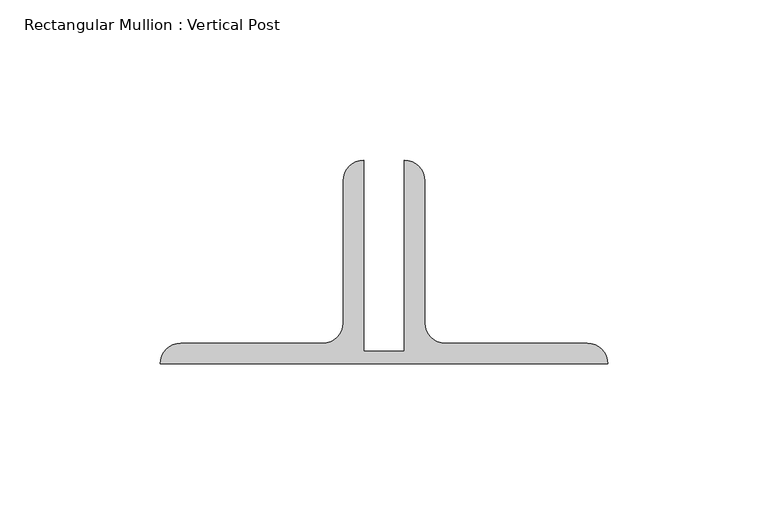
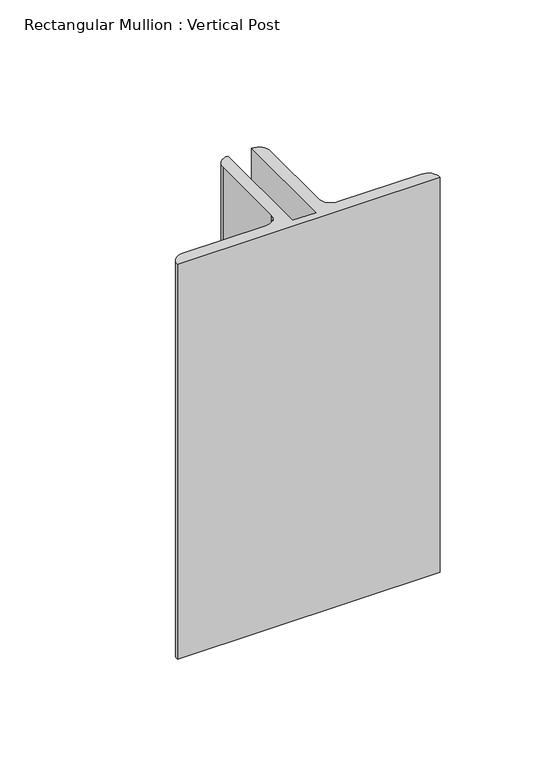
"""IFC4 building model written with IfcOpenShell, lengths in millimetres: member geometry, Rectangular Mullion : Vertical Post."""

from ifc_helpers import new_model, si_unit, point, frame, frame_2d, origin, place, context, project, spatial, polyline, circle_curve, trimmed, segment, composite_curve, outline, extrude, source, transform, mapped, element, save


def rectangular_mullion_vertical_post_d81d6a22(model_context):
    return source(origin(), model_context, "Body", "SweptSolid", [
        extrude(outline(composite_curve([segment(polyline([(-6.35, 22.9145205), (6.35, 22.9145205), (6.35, 82.55)]), True, "CONTINUOUS"), segment(trimmed(circle_curve(frame_2d((6.35, 76.2)), 6.35), [point((6.35, 82.55))], [point((12.7, 76.2))], False, "CARTESIAN"), True, "CONTINUOUS"), segment(polyline([(12.7, 76.2), (12.7, 31.75)]), True, "CONTINUOUS"), segment(trimmed(circle_curve(frame_2d((19.05, 31.75)), 6.35), [point((12.7, 31.75))], [point((19.05, 25.4))], True, "CARTESIAN"), True, "CONTINUOUS"), segment(polyline([(19.05, 25.4), (63.5, 25.4)]), True, "CONTINUOUS"), segment(trimmed(circle_curve(frame_2d((63.5, 19.05)), 6.35), [point((63.5, 25.4))], [point((69.85, 19.05))], False, "CARTESIAN"), True, "CONTINUOUS"), segment(polyline([(69.85, 19.05), (-69.85, 19.05)]), True, "CONTINUOUS"), segment(trimmed(circle_curve(frame_2d((-63.5, 19.05)), 6.35), [point((-69.85, 19.05))], [point((-63.5, 25.4))], False, "CARTESIAN"), True, "CONTINUOUS"), segment(polyline([(-63.5, 25.4), (-19.05, 25.4)]), True, "CONTINUOUS"), segment(trimmed(circle_curve(frame_2d((-19.05, 31.75)), 6.35), [point((-19.05, 25.4))], [point((-12.7, 31.75))], True, "CARTESIAN"), True, "CONTINUOUS"), segment(polyline([(-12.7, 31.75), (-12.7, 76.2)]), True, "CONTINUOUS"), segment(trimmed(circle_curve(frame_2d((-6.35, 76.2)), 6.35), [point((-12.7, 76.2))], [point((-6.35, 82.55))], False, "CARTESIAN"), True, "CONTINUOUS"), segment(polyline([(-6.35, 82.55), (-6.35, 22.9145205)]), True, "CONTINUOUS")], self_intersect=False)), frame((0.0, 0.0, -222.0889998), z_axis=(0.0, 0.0, 1.0), x_axis=(1.0, 0.0, 0.0)), (0.0, 0.0, 1.0), 222.0889998),
    ])


if __name__ == "__main__":
    model = new_model("IFC4")
    model_context = context("Model", 3, world=origin())
    ifc_project = project(units=[si_unit("LENGTHUNIT", "METRE", prefix="MILLI")], contexts=[model_context])
    site = spatial("IfcSite", under=ifc_project)
    building = spatial("IfcBuilding", under=site)
    placement = place(None, origin())
    rectangular_mullion_vertical_post_shape = rectangular_mullion_vertical_post_d81d6a22(model_context)
    element("IfcMember", 1, ObjectType="Rectangular Mullion : Vertical Post", at=placement, inside=building, context=model_context, shape_type="MappedRepresentation", body=[
        mapped(rectangular_mullion_vertical_post_shape, transform((0.0, 0.0, 0.0), x_axis=(1.0, 0.0, 0.0), y_axis=(0.0, 1.0, 0.0), z_axis=(0.0, 0.0, 1.0))),
    ])
    save(model, "model.ifc")

# Revit data of these elements
# Type "Rectangular Mullion : Vertical Post"
#   built-in parameter 1007351 = -0.0625 (stored number, unit not read)
#   built-in parameter 1007322 = 0.0126789 (stored number, unit not read)
#   built-in parameter 1007321 = 0.229167 (stored number, unit not read)
#   built-in parameter 1007320 = 0.229167 (stored number, unit not read)
# Element 1 (IfcMember, "Rectangular Mullion : Vertical Post")
#   Materials on its faces: "GATE POST: (2) BACK/BACK GALVANIZED ANGLES"
# Materials
#   "GATE POST: (2) BACK/BACK GALVANIZED ANGLES": class "Unassigned", colour RGB 211 211 211, transparency 0, Cost = 0
